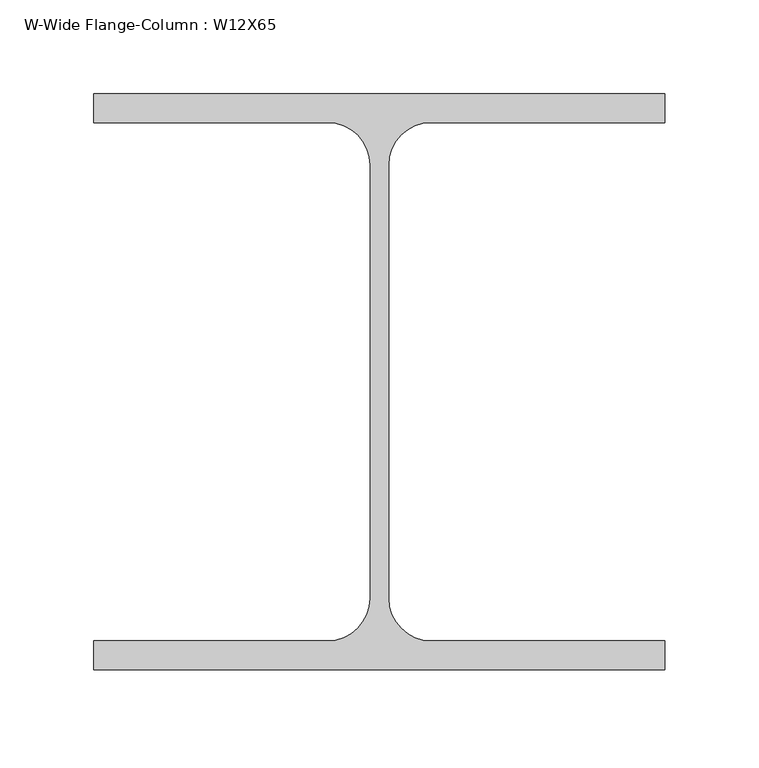
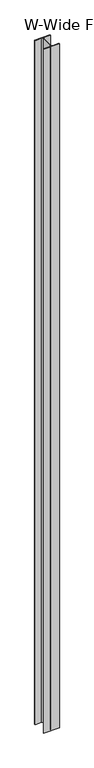
"""IFC4 building model written with IfcOpenShell, lengths in millimetres: column geometry, W-Wide Flange-Column : W12X65."""

from ifc_helpers import new_model, si_unit, point, frame, frame_2d, origin, place, context, project, spatial, polyline, circle_curve, trimmed, segment, composite_curve, outline, extrude, source, transform, mapped, element, save


def w_wide_flange_column_w12x65_25bd69bb(model_context):
    return source(origin(), model_context, "Body", "SweptSolid", [
        extrude(outline(composite_curve([segment(polyline([(152.4, 153.67), (152.4, 138.303), (27.686, 138.303)]), True, "CONTINUOUS"), segment(trimmed(circle_curve(frame_2d((27.686, 115.57)), 22.733), [point((27.686, 138.303))], [point((4.953, 115.57))], True, "CARTESIAN"), True, "CONTINUOUS"), segment(polyline([(4.953, 115.57), (4.953, -115.57)]), True, "CONTINUOUS"), segment(trimmed(circle_curve(frame_2d((27.686, -115.57)), 22.733), [point((4.953, -115.57))], [point((27.686, -138.303))], True, "CARTESIAN"), True, "CONTINUOUS"), segment(polyline([(27.686, -138.303), (152.4, -138.303), (152.4, -153.67), (-152.4, -153.67), (-152.4, -138.303), (-27.686, -138.303)]), True, "CONTINUOUS"), segment(trimmed(circle_curve(frame_2d((-27.686, -115.57)), 22.733), [point((-27.686, -138.303))], [point((-4.953, -115.57))], True, "CARTESIAN"), True, "CONTINUOUS"), segment(polyline([(-4.953, -115.57), (-4.953, 115.57)]), True, "CONTINUOUS"), segment(trimmed(circle_curve(frame_2d((-27.686, 115.57)), 22.733), [point((-4.953, 115.57))], [point((-27.686, 138.303))], True, "CARTESIAN"), True, "CONTINUOUS"), segment(polyline([(-27.686, 138.303), (-152.4, 138.303), (-152.4, 153.67), (152.4, 153.67)]), True, "CONTINUOUS")], self_intersect=False)), frame((0.0, 0.0, 9163.05), z_axis=(0.0, 0.0, 1.0), x_axis=(1.0, 0.0, 0.0)), (0.0, 0.0, 1.0), 14154.15),
    ])


if __name__ == "__main__":
    model = new_model("IFC4")
    model_context = context("Model", 3, world=origin())
    ifc_project = project(units=[si_unit("LENGTHUNIT", "METRE", prefix="MILLI")], contexts=[model_context])
    site = spatial("IfcSite", under=ifc_project)
    building = spatial("IfcBuilding", under=site)
    placement = place(None, origin())
    w_wide_flange_column_w12x65_shape = w_wide_flange_column_w12x65_25bd69bb(model_context)
    element("IfcColumn", 1, ObjectType="W-Wide Flange-Column : W12X65", at=placement, inside=building, context=model_context, shape_type="MappedRepresentation", body=[
        mapped(w_wide_flange_column_w12x65_shape, transform((0.0, 0.0, 0.0), x_axis=(1.0, 0.0, 0.0), y_axis=(0.0, 1.0, 0.0), z_axis=(0.0, 0.0, 1.0))),
    ])
    save(model, "model.ifc")

# Revit data of these elements
# Type "W-Wide Flange-Column : W12X65"
#   Assembly Code = "B10"
#   W = 65
#   bf = 1' - 0"
#   d = 1' - 0.1"
#   k = 0' - 1 1/2"
#   kr = 0' - 0.895"
#   tf = 0' - 0.605"
#   tw = 0' - 0.39"
#   A = 0.132639 SF
#   Structural Material [instance default] = Steel ASTM A992
# Element 1 (IfcColumn, "W-Wide Flange-Column : W12X65")
#   Materials on its faces: "Steel ASTM A992"
# Materials
#   "Steel ASTM A992": class "Metal", colour RGB 199 199 199, transparency 0, Description = "Structural steel 50ksi", Cost = 0
